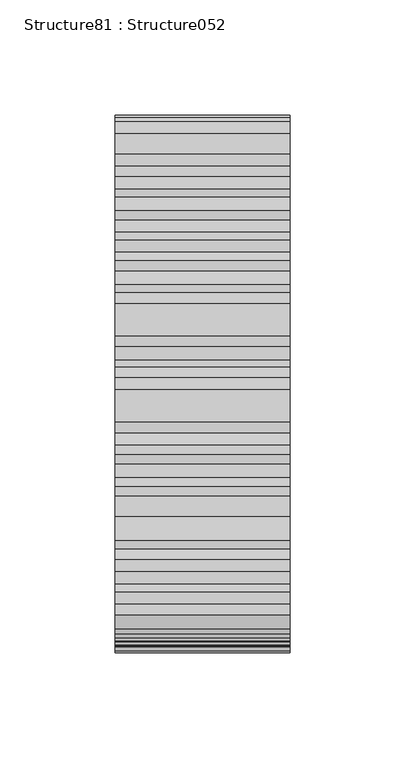
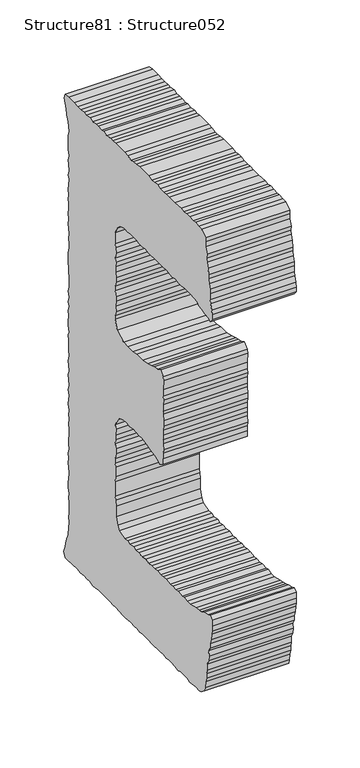
"""IFC4 building model written with IfcOpenShell, lengths in millimetres: proxy geometry, Structure81 : Structure052."""

from ifc_helpers import new_model, si_unit, frame, origin, place, context, project, spatial, polyline, outline, extrude, source, transform, mapped, element, save


def structure81_structure052_fde8bbe2(model_context):
    return source(origin(), model_context, "Body", "SweptSolid", [
        extrude(outline(polyline([(277340.8350089, 3552.242032), (277335.5751154, 3556.3417965), (277334.9733887, 3559.8671125), (277334.3941265, 3565.7094775), (277332.6322708, 3570.4109687), (277332.6322708, 3574.5107332), (277331.4512819, 3578.6104977), (277331.4512819, 3584.4689087), (277329.7134952, 3588.5702778), (277328.5325063, 3593.8285667), (277329.134233, 3598.5284533), (277326.7722551, 3602.6298224), (277327.3739818, 3606.7295868), (277325.5912662, 3611.4134274), (277325.0103994, 3617.2718384), (277323.8294105, 3620.7971545), (277323.8294105, 3625.472972), (277323.8294105, 3631.3410106), (277327.3739818, 3633.6821286), (277330.2702929, 3632.5155811), (277336.1543776, 3631.3410106), (277340.2541421, 3629.5984101), (277344.3555112, 3628.4158166), (277349.0361425, 3627.8397636), (277358.418265, 3625.472972), (277363.0988963, 3625.472972), (277367.777923, 3626.6571701), (277371.3000299, 3625.472972), (277377.1600455, 3626.6571701), (277381.2838791, 3625.472972), (277385.9420459, 3626.0554434), (277390.0418104, 3625.472972), (277395.9258951, 3626.6571701), (277401.1857886, 3626.0554434), (277405.2855531, 3625.472972), (277409.3869222, 3626.6571701), (277414.6676756, 3625.472972), (277418.7690447, 3626.0554434), (277423.449676, 3625.472972), (277428.1287027, 3626.6571701), (277434.0127874, 3625.472972), (277439.2726809, 3626.0554434), (277443.9517076, 3625.472972), (277447.4738145, 3626.6571701), (277453.3354347, 3625.472972), (277456.855937, 3626.6571701), (277461.5365683, 3626.0554434), (277470.3394286, 3628.4158166), (277472.6564775, 3631.915459), (277475.0200599, 3638.9580681), (277475.0200599, 3648.9258713), (277475.5993221, 3654.1841602), (277476.1785843, 3657.7014533), (277476.1785843, 3671.7690209), (277475.5993221, 3677.0449605), (277475.5993221, 3685.8285655), (277476.1785843, 3689.3458585), (277476.1785843, 3694.029699), (277475.0200599, 3699.3136616), (277475.0200599, 3704.0135482), (277476.1785843, 3708.087639), (277475.5993221, 3712.2146818), (277475.5993221, 3716.8985223), (277475.0200599, 3722.7312597), (277476.1785843, 3726.2742264), (277472.0996797, 3733.8736333), (277470.3394286, 3736.2163558), (277462.7175572, 3739.1592005), (277457.4127348, 3739.1592005), (277453.3354347, 3738.5574738), (277447.4738145, 3739.7416719), (277443.9517076, 3739.1592005), (277438.091692, 3738.5574738), (277434.0127874, 3739.1592005), (277425.2099271, 3737.400554), (277420.5068314, 3735.6146291), (277414.6676756, 3734.47536), (277410.5679111, 3733.2991849), (277406.4440776, 3730.9323932), (277400.6065264, 3734.47536), (277400.6065264, 3739.7416719), (277401.1857886, 3744.4158848), (277400.0047997, 3748.5429276), (277401.1857886, 3753.8012165), (277400.6065264, 3757.8753073), (277401.1857886, 3762.0023501), (277401.1857886, 3766.684586), (277400.0047997, 3771.3860772), (277400.0047997, 3776.6427615), (277401.1857886, 3781.9299333), (277400.6065264, 3785.4456218), (277401.1857886, 3791.3056374), (277400.0047997, 3795.960595), (277400.6065264, 3799.5051664), (277401.1857886, 3805.3459267), (277400.0047997, 3814.7296538), (277400.6065264, 3818.2309008), (277405.2855531, 3822.348316), (277409.9886489, 3820.015221), (277415.2485424, 3818.8310229), (277419.3483069, 3817.6741031), (277425.2099271, 3815.9154565), (277433.4110607, 3814.148787), (277442.7707187, 3814.148787), (277448.6548034, 3812.9726119), (277456.855937, 3812.9726119), (277462.7175572, 3813.5743386), (277473.2357397, 3818.8310229), (277476.1785843, 3827.6162325), (277476.1785843, 3831.1575946), (277475.0200599, 3835.8334121), (277475.5993221, 3840.5172527), (277475.0200599, 3845.8012153), (277475.0200599, 3849.8753061), (277476.1785843, 3855.1769193), (277476.1785843, 3859.2606378), (277475.0200599, 3863.9332461), (277475.0200599, 3868.0618934), (277475.5993221, 3873.3185778), (277475.5993221, 3878.5784713), (277475.0200599, 3883.2863809), (277476.1785843, 3886.2051565), (277475.0200599, 3891.5067697), (277475.5993221, 3896.763454), (277476.1785843, 3900.2887701), (277476.1785843, 3910.8310217), (277473.2357397, 3916.6653636), (277469.7377019, 3920.7908018), (277462.1158305, 3923.7079727), (277456.855937, 3923.1319197), (277452.1544458, 3923.7079727), (277442.7707187, 3923.7079727), (277439.2726809, 3923.1319197), (277433.4110607, 3922.5494483), (277429.3096916, 3923.7079727), (277424.0289382, 3922.5494483), (277419.9275691, 3922.5494483), (277415.2485424, 3923.1319197), (277401.1857886, 3923.1319197), (277395.3241684, 3923.7079727), (277390.6210726, 3922.5494483), (277386.5437726, 3922.5494483), (277381.8631413, 3923.7079727), (277377.1600455, 3922.5494483), (277371.9017566, 3922.5494483), (277367.777923, 3923.7079727), (277358.418265, 3923.7079727), (277347.8551536, 3922.5494483), (277344.9347734, 3920.2067257), (277340.2541421, 3919.6066036), (277335.5751154, 3918.4480792), (277330.2702929, 3917.8479571), (277327.3739818, 3915.5068392), (277323.8294105, 3919.6066036), (277323.8294105, 3924.2888396), (277324.4311372, 3928.4158823), (277326.1929929, 3933.6741713), (277326.7722551, 3937.1930689), (277327.3739818, 3942.4770315), (277327.3739818, 3946.5511223), (277328.5325063, 3951.2606365), (277329.7134952, 3955.360401), (277329.134233, 3959.4617701), (277330.2702929, 3965.3201811), (277332.0530085, 3969.994394), (277332.6322708, 3973.5197101), (277332.0530085, 3977.6194746), (277334.3941265, 3983.4794902), (277334.3941265, 3988.1633307), (277334.3941265, 3991.6806238), (277340.2541421, 3996.390138), (277344.9347734, 3996.390138), (277350.2171314, 3996.9645864), (277353.7151692, 3996.390138), (277358.9975272, 3996.9645864), (277364.2798852, 3996.9645864), (277368.9589119, 3995.7803883), (277372.4810188, 3996.9645864), (277383.0216657, 3995.7803883), (277391.8020615, 3995.7803883), (277395.9258951, 3996.390138), (277400.0047997, 3995.7803883), (277405.8648153, 3995.7803883), (277409.9886489, 3996.9645864), (277414.0659489, 3996.9645864), (277419.3483069, 3995.7803883), (277424.0289382, 3996.9645864), (277438.091692, 3996.9645864), (277443.3724454, 3996.390138), (277448.0755412, 3995.7803883), (277450.9718523, 3995.7803883), (277456.855937, 3996.390138), (277461.5365683, 3996.9645864), (277475.5993221, 3996.9645864), (277480.2783488, 3996.390138), (277483.8004557, 3996.9645864), (277489.6620759, 3995.7803883), (277494.3635671, 3996.9645864), (277497.8632095, 3995.7803883), (277503.1214984, 3996.390138), (277506.6436053, 3996.390138), (277511.9259633, 3995.7803883), (277516.0257278, 3996.9645864), (277521.887348, 3995.7803883), (277525.3853858, 3996.390138), (277530.6902083, 3995.7803883), (277535.3708396, 3995.7803883), (277540.6291285, 3996.390138), (277549.4111289, 3996.390138), (277554.7143468, 3995.7803883), (277556.453738, 3991.6806238), (277554.7143468, 3987.5792547), (277553.5333579, 3982.8793681), (277552.9540956, 3977.6194746), (277550.0128556, 3972.3627903), (277548.8318667, 3964.1343784), (277550.0128556, 3958.8776941), (277550.0128556, 3945.9766739), (277548.8318667, 3940.718385), (277550.0128556, 3935.4328178), (277549.4111289, 3931.9058971), (277548.8318667, 3926.0490907), (277550.0128556, 3921.3748778), (277548.8318667, 3917.8479571), (277550.0128556, 3907.3313793), (277549.4111289, 3902.6314927), (277550.0128556, 3897.9476522), (277549.4111289, 3894.4030808), (277549.4111289, 3889.7208449), (277550.0128556, 3884.4609514), (277549.4111289, 3879.7610648), (277550.0128556, 3874.5043805), (277548.8318667, 3866.3032469), (277549.4111289, 3861.0192843), (277548.8318667, 3855.7353217), (277548.8318667, 3852.2340747), (277550.0128556, 3846.9757858), (277550.0128556, 3836.9919366), (277549.4111289, 3832.8921721), (277549.4111289, 3828.2163546), (277548.8318667, 3824.1149855), (277548.8318667, 3814.7296538), (277550.0128556, 3810.0474179), (277548.8318667, 3804.7730829), (277550.0128556, 3799.5051664), (277548.8318667, 3795.960595), (277550.0128556, 3791.3056374), (277549.4111289, 3786.6298199), (277550.0128556, 3781.3282066), (277550.0128556, 3777.2444882), (277548.8318667, 3771.3860772), (277550.0128556, 3767.8607611), (277549.4111289, 3762.5848215), (277549.4111289, 3753.2171405), (277548.8318667, 3748.5429276), (277550.0128556, 3743.2332913), (277549.4111289, 3739.1592005), (277548.8318667, 3733.8736333), (277550.0128556, 3730.3563402), (277549.4111289, 3725.0996559), (277548.8318667, 3720.4158154), (277550.0128556, 3715.1302482), (277548.8318667, 3710.4560353), (277549.4111289, 3706.9130685), (277550.0128556, 3701.6547796), (277548.8318667, 3696.3884676), (277549.4111289, 3692.2710525), (277548.8318667, 3687.587212), (277549.4111289, 3682.8857208), (277548.8318667, 3677.6274319), (277548.8318667, 3672.9435914), (277549.4111289, 3668.8261762), (277549.4111289, 3663.5598643), (277548.8318667, 3658.8840468), (277550.0128556, 3654.7842823), (277549.4111289, 3650.1004418), (277550.0128556, 3645.4262289), (277549.4111289, 3641.2991861), (277548.8318667, 3636.0408972), (277549.4111289, 3630.7392839), (277550.0128556, 3626.6571701), (277550.0128556, 3621.3732075), (277548.8318667, 3616.69739), (277549.4111289, 3612.0135494), (277548.8318667, 3607.3393366), (277548.8318667, 3597.9540049), (277549.4111289, 3593.8285667), (277548.8318667, 3588.5702778), (277549.4111289, 3583.8864372), (277550.5921178, 3575.6853037), (277552.352369, 3570.9854171), (277554.1126201, 3565.7094775), (277554.7143468, 3561.6257591), (277557.634727, 3555.7416744), (277554.7143468, 3551.0658569), (277550.0128556, 3551.0658569), (277544.7304976, 3551.6675836), (277535.3708396, 3551.6675836), (277531.2694705, 3551.0658569), (277525.3853858, 3551.6675836), (277520.7063591, 3551.0658569), (277516.6274545, 3551.6675836), (277511.9259633, 3550.4833855), (277507.245332, 3550.4833855), (277502.5422362, 3551.6675836), (277484.3797179, 3551.6675836), (277479.6990866, 3551.0658569), (277475.5993221, 3551.6675836), (277465.0346061, 3550.4833855), (277460.9573061, 3550.4833855), (277455.6749481, 3551.0658569), (277452.1544458, 3551.6675836), (277446.8945523, 3551.0658569), (277442.213921, 3551.0658569), (277438.091692, 3550.4833855), (277432.8317985, 3551.6675836), (277423.449676, 3551.6675836), (277419.9275691, 3551.0658569), (277405.8648153, 3551.0658569), (277401.1857886, 3551.6675836), (277396.5051573, 3550.4833855), (277392.4037882, 3551.6675836), (277387.7247615, 3551.6675836), (277383.0216657, 3551.0658569), (277377.1600455, 3550.4833855), (277373.6620077, 3551.6675836), (277363.0988963, 3551.6675836), (277358.9975272, 3550.4833855), (277349.6378692, 3551.6675836), (277344.3555112, 3551.0658569), (277340.8350089, 3552.242032)])), frame((-59031.6926606, 0.0, 0.0), z_axis=(1.0, 0.0, 0.0), x_axis=(0.0, 1.0, 0.0)), (0.0, 0.0, 1.0), 76.2),
    ])


if __name__ == "__main__":
    model = new_model("IFC4")
    model_context = context("Model", 3, world=origin())
    ifc_project = project(units=[si_unit("LENGTHUNIT", "METRE", prefix="MILLI")], contexts=[model_context])
    site = spatial("IfcSite", under=ifc_project)
    building = spatial("IfcBuilding", under=site)
    placement = place(None, origin())
    structure81_structure052_shape = structure81_structure052_fde8bbe2(model_context)
    element("IfcBuildingElementProxy", 1, Name="Structure81 : Structure052", ObjectType="Structure81 : Structure052", at=placement, inside=building, context=model_context, shape_type="MappedRepresentation", body=[
        mapped(structure81_structure052_shape, transform((0.0, 0.0, 0.0), x_axis=(1.0, 0.0, 0.0), y_axis=(0.0, 1.0, 0.0), z_axis=(0.0, 0.0, 1.0))),
    ])
    save(model, "model.ifc")

# Revit data of these elements
# Type "Structure81 : Structure052"
#   NameOverride = "Structure052"
# Element 1 (IfcBuildingElementProxy, "Structure81 : Structure052")
#   Materials on its faces: "BRUSHED ALUM. LETTERING"
# Materials
#   "BRUSHED ALUM. LETTERING": class "Unassigned", colour RGB 169 181 186, transparency 0, Cost = 0
